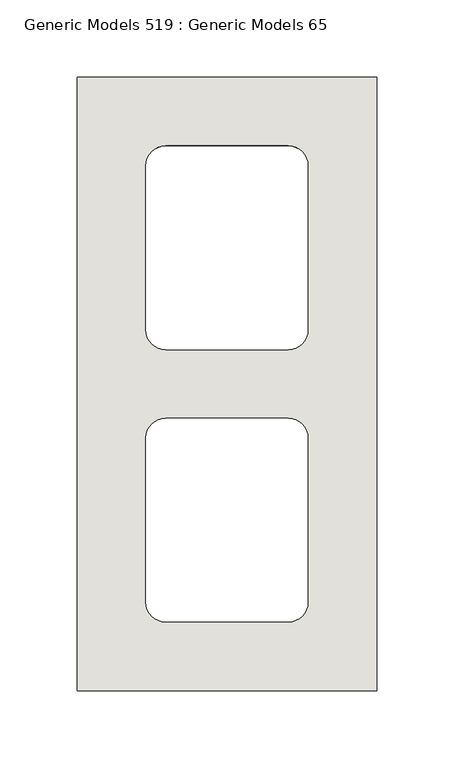
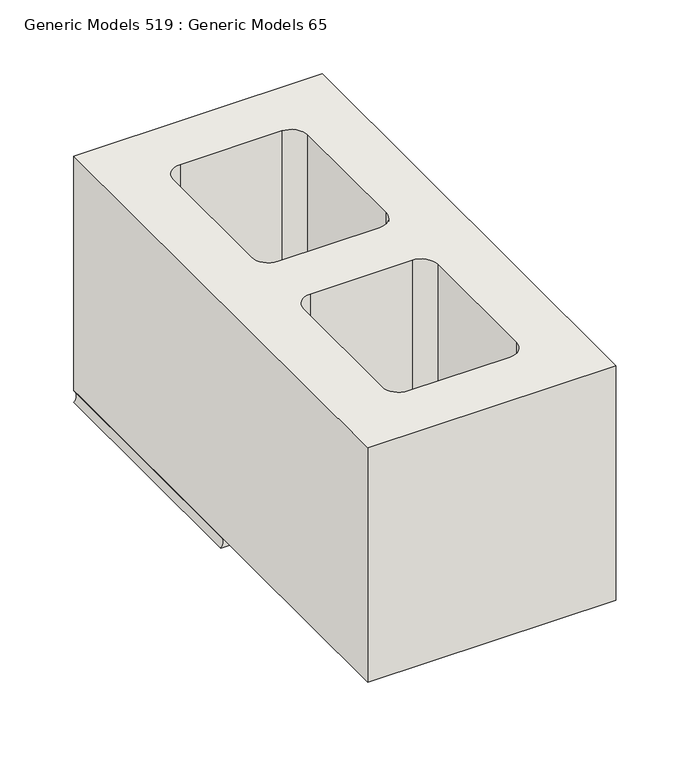
"""IFC4 building model written with IfcOpenShell, lengths in millimetres: wall geometry, Generic Models 519 : Generic Models 65."""

from ifc_helpers import new_model, si_unit, point, frame, frame_2d, origin, place, context, project, spatial, polyline, circle_curve, trimmed, segment, composite_curve, outline, extrude, source, transform, mapped, element, save
from ifc_brep_helpers import plane_surface, revolved_surface, advanced_brep


def generic_models_519_generic_models_65_fed30d2b(model_context):
    return source(origin(), model_context, "Body", "SolidModel", [
        advanced_brep(
        [(428979.0125, 503.2375, 1431.925), (428785.3375, 503.2375, 1431.925), (428785.3375, 503.2375, 1422.4), (428979.0125, 503.2375, 1422.4), (428979.0125, 701.675, 1431.925), (428979.0125, 701.675, 1422.4), (428785.3375, 701.675, 1422.4), (428785.3375, 701.675, 1431.925), (428934.5625, 538.1625, 1431.925), (428921.8625, 525.4625, 1431.925), (428842.4875, 525.4625, 1431.925), (428829.7875, 538.1625, 1431.925), (428829.7875, 644.525, 1431.925), (428842.4875, 657.225, 1431.925), (428921.8625, 657.225, 1431.925), (428934.5625, 644.525, 1431.925), (428921.8625, 525.4625, 1422.4), (428934.5625, 538.1625, 1422.4), (428842.4875, 525.4625, 1422.4), (428829.7875, 538.1625, 1422.4), (428829.7875, 644.525, 1422.4), (428842.4875, 657.225, 1422.4), (428921.8625, 657.225, 1422.4), (428934.5625, 644.525, 1422.4)],
        [
            (0, 1),
            (1, 2, circle_curve(frame((428780.4545028, 503.2375, 1427.1625), z_axis=(0.0, 1.0, 0.0), x_axis=(1.0, 0.0, 0.0)), 6.8209287)),
            (2, 3),
            (3, 0, circle_curve(frame((428983.8954972, 503.2375, 1427.1625), z_axis=(0.0, 1.0, 0.0), x_axis=(-1.0, 0.0, 0.0)), 6.8209287)),
            (4, 5, circle_curve(frame((428983.8954972, 701.675, 1427.1625), z_axis=(0.0, -1.0, 0.0), x_axis=(-1.0, 0.0, 0.0)), 6.8209287)),
            (5, 6),
            (6, 7, circle_curve(frame((428780.4545028, 701.675, 1427.1625), z_axis=(0.0, -1.0, 0.0), x_axis=(1.0, 0.0, 0.0)), 6.8209287)),
            (7, 4),
            (0, 4),
            (7, 1),
            (8, 9, circle_curve(frame((428921.8625, 538.1625, 1431.925), z_axis=(0.0, 0.0, -1.0), x_axis=(-1.0, 0.0, 0.0)), 12.7)),
            (9, 10),
            (10, 11, circle_curve(frame((428842.4875, 538.1625, 1431.925), z_axis=(0.0, 0.0, -1.0), x_axis=(-1.0, 0.0, 0.0)), 12.7)),
            (11, 12),
            (12, 13, circle_curve(frame((428842.4875, 644.525, 1431.925), z_axis=(0.0, 0.0, -1.0), x_axis=(-1.0, 0.0, 0.0)), 12.7)),
            (13, 14),
            (14, 15, circle_curve(frame((428921.8625, 644.525, 1431.925), z_axis=(0.0, 0.0, -1.0), x_axis=(-1.0, 0.0, 0.0)), 12.7)),
            (15, 8),
            (16, 9),
            (8, 17),
            (17, 16, circle_curve(frame((428921.8625, 538.1625, 1422.4), z_axis=(0.0, 0.0, -1.0), x_axis=(-1.0, 0.0, 0.0)), 12.7)),
            (16, 18),
            (18, 10),
            (18, 19, circle_curve(frame((428842.4875, 538.1625, 1422.4), z_axis=(0.0, 0.0, -1.0), x_axis=(-1.0, 0.0, 0.0)), 12.7)),
            (19, 11),
            (19, 20),
            (20, 12),
            (20, 21, circle_curve(frame((428842.4875, 644.525, 1422.4), z_axis=(0.0, 0.0, -1.0), x_axis=(-1.0, 0.0, 0.0)), 12.7)),
            (21, 13),
            (21, 22),
            (22, 14),
            (22, 23, circle_curve(frame((428921.8625, 644.525, 1422.4), z_axis=(0.0, 0.0, -1.0), x_axis=(-1.0, 0.0, 0.0)), 12.7)),
            (23, 15),
            (23, 17),
            (6, 2),
            (5, 3),
        ],
        [
            plane_surface(frame((428882.175, 503.2375, 1432.321875), z_axis=(0.0, -1.0, 0.0), x_axis=(0.0, 0.0, 1.0))),
            plane_surface(frame((428882.175, 701.675, 1432.321875), z_axis=(0.0, 1.0, 0.0), x_axis=(0.0, 0.0, 1.0))),
            plane_surface(frame((428979.0125, 503.2375, 1431.925), z_axis=(0.0, 0.0, 1.0), x_axis=(0.0, 1.0, 0.0))),
            revolved_surface(polyline([(428909.1625, 538.1625, 1431.925), (428909.1625, 538.1625, 1422.4)]), (428921.8625, 538.1625, 1616.075), (0.0, 0.0, 1.0)),
            plane_surface(frame((428842.4875, 525.4625, 1616.075), z_axis=(0.0, 1.0, 0.0), x_axis=(0.0, 0.0, -1.0))),
            revolved_surface(polyline([(428829.7875, 538.1625, 1431.925), (428829.7875, 538.1625, 1422.4)]), (428842.4875, 538.1625, 1616.075), (0.0, 0.0, 1.0)),
            plane_surface(frame((428829.7875, 644.525, 1616.075), z_axis=(1.0, 0.0, 0.0), x_axis=(0.0, 0.0, -1.0))),
            revolved_surface(polyline([(428829.7875, 644.525, 1431.925), (428829.7875, 644.525, 1422.4)]), (428842.4875, 644.525, 1616.075), (0.0, 0.0, 1.0)),
            plane_surface(frame((428921.8625, 657.225, 1616.075), z_axis=(0.0, -1.0, 0.0), x_axis=(0.0, 0.0, -1.0))),
            revolved_surface(polyline([(428909.1625, 644.525, 1431.925), (428909.1625, 644.525, 1422.4)]), (428921.8625, 644.525, 1616.075), (0.0, 0.0, 1.0)),
            plane_surface(frame((428934.5625, 538.1625, 1616.075), z_axis=(-1.0, 0.0, 0.0), x_axis=(0.0, 0.0, -1.0))),
            revolved_surface(polyline([(428787.2754315, 701.675, 1427.1625), (428787.2754315, 503.2375, 1427.1625)]), (428780.4545028, 503.2375, 1427.1625), (0.0, 1.0, 0.0)),
            plane_surface(frame((428785.3375, 503.2375, 1422.4), z_axis=(0.0, 0.0, -1.0), x_axis=(0.0, 1.0, 0.0))),
            revolved_surface(polyline([(428977.07456850004, 701.675, 1427.1625), (428977.07456850004, 503.2375, 1427.1625)]), (428983.8954972, 503.2375, 1427.1625), (0.0, 1.0, 0.0)),
        ],
        [
            (0, [[1, 2, 3, 4]]),
            (1, [[5, 6, 7, 8]]),
            (2, [[-1, 9, -8, 10], [11, 12, 13, 14, 15, 16, 17, 18]]),
            (3, [[19, -11, 20, 21]]),
            (4, [[-19, 22, 23, -12]]),
            (5, [[-23, 24, 25, -13]]),
            (6, [[-25, 26, 27, -14]]),
            (7, [[-27, 28, 29, -15]]),
            (8, [[-29, 30, 31, -16]]),
            (9, [[-31, 32, 33, -17]]),
            (10, [[-33, 34, -20, -18]]),
            (11, [[-2, -10, -7, 35]]),
            (12, [[-3, -35, -6, 36], [-21, -34, -32, -30, -28, -26, -24, -22]]),
            (13, [[-4, -36, -5, -9]]),
        ],
    ),
        extrude(outline(polyline([(428979.0125, 304.8), (428785.3375, 304.8), (428785.3375, 701.675), (428979.0125, 701.675), (428979.0125, 304.8)]), holes=[composite_curve([segment(polyline([(428934.5625, 538.1625), (428934.5625, 644.525)]), True, "CONTINUOUS"), segment(trimmed(circle_curve(frame_2d((428921.8625, 644.525)), 12.7), [point((428934.5625, 644.525))], [point((428921.8625, 657.225))], True, "CARTESIAN"), True, "CONTINUOUS"), segment(polyline([(428921.8625, 657.225), (428842.4875, 657.225)]), True, "CONTINUOUS"), segment(trimmed(circle_curve(frame_2d((428842.4875, 644.525)), 12.7), [point((428842.4875, 657.225))], [point((428829.7875, 644.525))], True, "CARTESIAN"), True, "CONTINUOUS"), segment(polyline([(428829.7875, 644.525), (428829.7875, 538.1625)]), True, "CONTINUOUS"), segment(trimmed(circle_curve(frame_2d((428842.4875, 538.1625)), 12.7), [point((428829.7875, 538.1625))], [point((428842.4875, 525.4625))], True, "CARTESIAN"), True, "CONTINUOUS"), segment(polyline([(428842.4875, 525.4625), (428921.8625, 525.4625)]), True, "CONTINUOUS"), segment(trimmed(circle_curve(frame_2d((428921.8625, 538.1625)), 12.7), [point((428921.8625, 525.4625))], [point((428934.5625, 538.1625))], True, "CARTESIAN"), True, "CONTINUOUS")], self_intersect=False), composite_curve([segment(polyline([(428829.7875, 468.3125), (428829.7875, 361.95)]), True, "CONTINUOUS"), segment(trimmed(circle_curve(frame_2d((428842.4875, 361.95)), 12.7), [point((428829.7875, 361.95))], [point((428842.4875, 349.25))], True, "CARTESIAN"), True, "CONTINUOUS"), segment(polyline([(428842.4875, 349.25), (428921.8625, 349.25)]), True, "CONTINUOUS"), segment(trimmed(circle_curve(frame_2d((428921.8625, 361.95)), 12.7), [point((428921.8625, 349.25))], [point((428934.5625, 361.95))], True, "CARTESIAN"), True, "CONTINUOUS"), segment(polyline([(428934.5625, 361.95), (428934.5625, 468.3125)]), True, "CONTINUOUS"), segment(trimmed(circle_curve(frame_2d((428921.8625, 468.3125)), 12.7), [point((428934.5625, 468.3125))], [point((428921.8625, 481.0125))], True, "CARTESIAN"), True, "CONTINUOUS"), segment(polyline([(428921.8625, 481.0125), (428842.4875, 481.0125)]), True, "CONTINUOUS"), segment(trimmed(circle_curve(frame_2d((428842.4875, 468.3125)), 12.7), [point((428842.4875, 481.0125))], [point((428829.7875, 468.3125))], True, "CARTESIAN"), True, "CONTINUOUS")], self_intersect=False)]), frame((0.0, 0.0, 1431.925), z_axis=(0.0, 0.0, 1.0), x_axis=(1.0, 0.0, 0.0)), (0.0, 0.0, 1.0), 193.675),
    ])


if __name__ == "__main__":
    model = new_model("IFC4")
    model_context = context("Model", 3, world=origin())
    ifc_project = project(units=[si_unit("LENGTHUNIT", "METRE", prefix="MILLI")], contexts=[model_context])
    site = spatial("IfcSite", under=ifc_project)
    building = spatial("IfcBuilding", under=site)
    placement = place(None, origin())
    generic_models_519_generic_models_65_shape = generic_models_519_generic_models_65_fed30d2b(model_context)
    element("IfcWall", 1, ObjectType="Generic Models 519 : Generic Models 65", at=placement, inside=building, context=model_context, shape_type="MappedRepresentation", body=[
        mapped(generic_models_519_generic_models_65_shape, transform((0.0, 0.0, 0.0), x_axis=(1.0, 0.0, 0.0), y_axis=(0.0, 1.0, 0.0), z_axis=(0.0, 0.0, 1.0))),
    ])
    save(model, "model.ifc")

# Revit data of these elements
# Element 1 (IfcWall, "Generic Models 519 : Generic Models 65")
#   Materials on its faces: "CMU (SEE 'WALL TAG' FOR SIZE)", "MORTAR JOINT"
# Materials
#   "CMU (SEE 'WALL TAG' FOR SIZE)": class "Masonry", colour RGB 203 203 199, transparency 0, Description = "Concrete masonry units", Cost = 0
#   "MORTAR JOINT": class "Generic", colour RGB 120 120 120, transparency 0, Cost = 0
